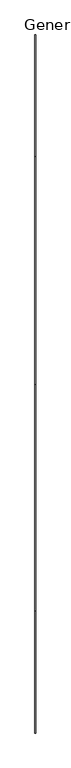
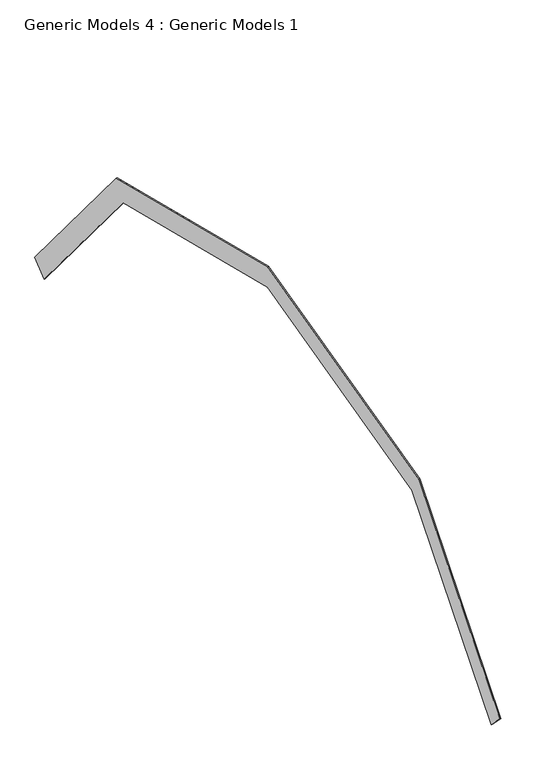
"""IFC4 building model written with IfcOpenShell, lengths in millimetres: proxy geometry, Generic Models 4 : Generic Models 1."""

from ifc_helpers import new_model, si_unit, frame, origin, place, context, project, spatial, polyline, outline, extrude, source, transform, mapped, element, save


def generic_models_4_generic_models_1_4f2df183(model_context):
    return source(origin(), model_context, "Body", "SweptSolid", [
        extrude(outline(polyline([(11606.2878096, 2984.3405795), (10019.9980933, 4887.8882391), (7109.4138362, 5615.5343034), (4198.7953154, 4887.8796732), (2604.5089175, 2974.7359957), (2431.2242181, 3148.0206952), (4062.7194377, 5105.8149588), (7110.1288453, 5867.6673107), (10157.5382529, 5105.8149588), (11793.7171223, 3142.4003155), (11606.2878096, 2984.3405795)])), frame((29947.3870052, 0.0, 0.0), z_axis=(1.0, 0.0, 0.0), x_axis=(0.0, 1.0, 0.0)), (0.0, 0.0, 1.0), 13.5023771),
    ])


if __name__ == "__main__":
    model = new_model("IFC4")
    model_context = context("Model", 3, world=origin())
    ifc_project = project(units=[si_unit("LENGTHUNIT", "METRE", prefix="MILLI")], contexts=[model_context])
    site = spatial("IfcSite", under=ifc_project)
    building = spatial("IfcBuilding", under=site)
    placement = place(None, origin())
    generic_models_4_generic_models_1_shape = generic_models_4_generic_models_1_4f2df183(model_context)
    element("IfcBuildingElementProxy", 1, Name="Generic Models 4 : Generic Models 1", ObjectType="Generic Models 4 : Generic Models 1", at=placement, inside=building, context=model_context, shape_type="MappedRepresentation", body=[
        mapped(generic_models_4_generic_models_1_shape, transform((0.0, 0.0, 0.0), x_axis=(1.0, 0.0, 0.0), y_axis=(0.0, 1.0, 0.0), z_axis=(0.0, 0.0, 1.0))),
    ])
    save(model, "model.ifc")
